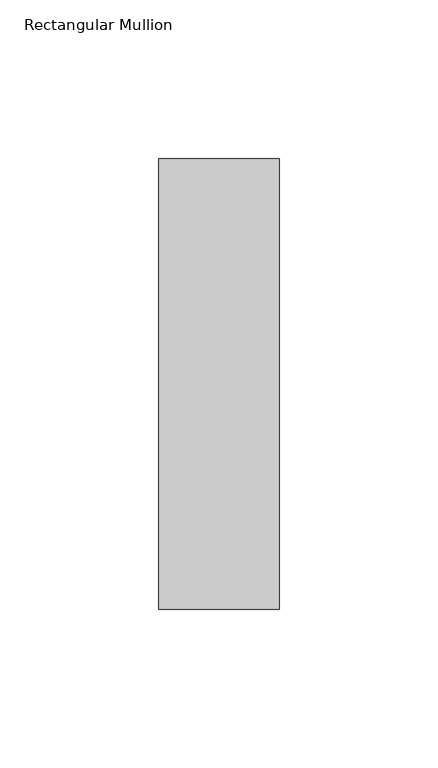
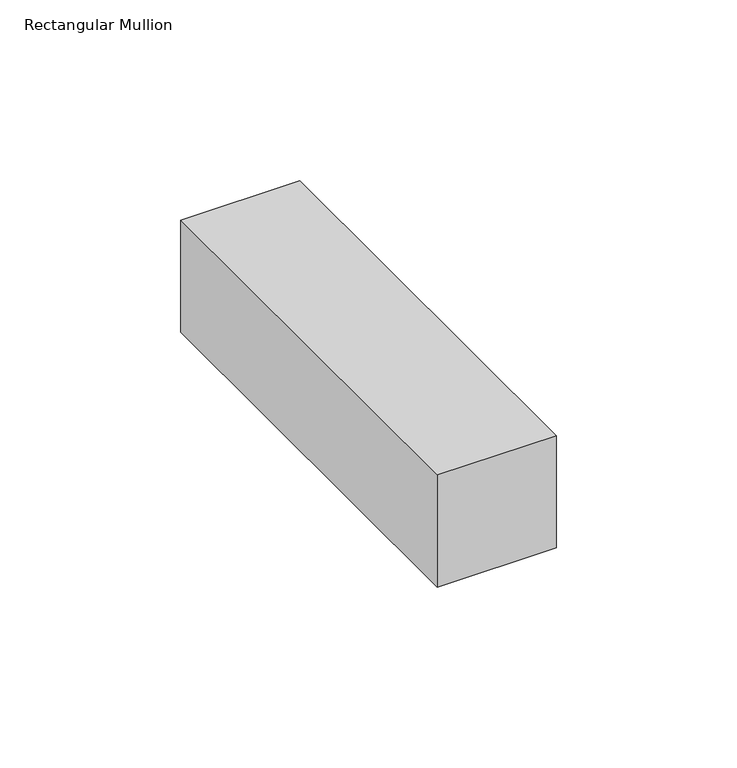
"""IFC4 building model written with IfcOpenShell, lengths in millimetres: member geometry, Rectangular Mullion : NLRS_21_CWM_hsb-regel 38x142_gen_rsf."""

from ifc_helpers import new_model, si_unit, frame, origin, place, context, project, spatial, polyline, outline, extrude, source, transform, mapped, element, save


def rectangular_mullion_a2f1b024(model_context):
    return source(origin(), model_context, "Body", "SweptSolid", [
        extrude(outline(polyline([(0.0, -71.0), (-38.0, -71.0), (-38.0, 71.0), (0.0, 71.0), (0.0, -71.0)])), frame((0.0, 0.0, -38.0), z_axis=(0.0, 0.0, 1.0), x_axis=(1.0, 0.0, 0.0)), (0.0, 0.0, 1.0), 38.0),
    ])


if __name__ == "__main__":
    model = new_model("IFC4")
    model_context = context("Model", 3, world=origin())
    ifc_project = project(units=[si_unit("LENGTHUNIT", "METRE", prefix="MILLI")], contexts=[model_context])
    site = spatial("IfcSite", under=ifc_project)
    building = spatial("IfcBuilding", under=site)
    placement = place(None, origin())
    rectangular_mullion_shape = rectangular_mullion_a2f1b024(model_context)
    element("IfcMember", 1, ObjectType="Rectangular Mullion : NLRS_21_CWM_hsb-regel 38x142_gen_rsf", at=placement, inside=building, context=model_context, shape_type="MappedRepresentation", body=[
        mapped(rectangular_mullion_shape, transform((0.0, 0.0, 0.0), x_axis=(1.0, 0.0, 0.0), y_axis=(0.0, 1.0, 0.0), z_axis=(0.0, 0.0, 1.0))),
    ])
    save(model, "model.ifc")

# Revit data of these elements
# Type "Rectangular Mullion : NLRS_21_CWM_hsb-regel 38x142_gen_rsf"
#   Export Type to IFC As = "IfcWall"
#   Type IfcGUID = "07M7mRoiH1CR8m_RSKIwpF"
#   Assembly Code = "21.10"
#   built-in parameter 1007322 = 0.465879 (stored number, unit not read)
#   built-in parameter 1007321 = 0.062336 (stored number, unit not read)
#   built-in parameter 1007320 = 0.062336 (stored number, unit not read)
# Element 1 (IfcMember, "Rectangular Mullion : NLRS_21_CWM_hsb-regel 38x142_gen_rsf")
#   Materials on its faces: "NLRS_i2_hout naaldhout vuren_gen_rsf"
# Materials
#   "NLRS_i2_hout naaldhout vuren_gen_rsf": class "I - Hout", colour RGB 234 199 147, transparency 0, Keynote = "i2", Manufacturer = "Revit Standards Foundation", URL = "www.revitstandards.org", Description = "hout vuren", Cost = 0
